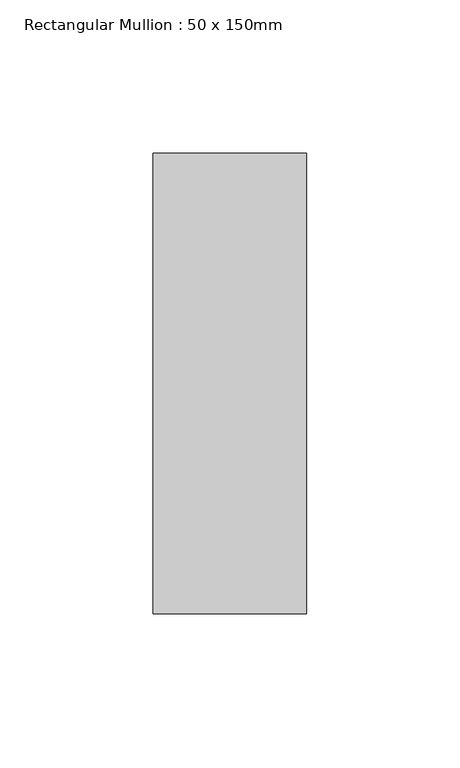
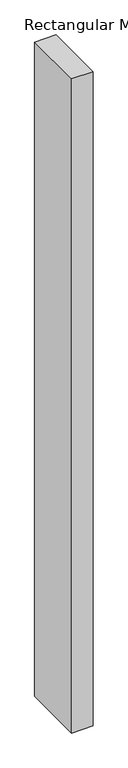
"""IFC4 building model written with IfcOpenShell, lengths in millimetres: member geometry, Rectangular Mullion : 50 x 150mm."""

import ifcopenshell
import ifcopenshell.guid

model = None  # the IFC model being written
_history = None  # IfcOwnerHistory: only IFC2X3 demands one
_inside = {}  # id of a spatial element -> (the spatial element, [elements in it])
_under = {}  # id of a project, library or spatial element -> (it, [spatial elements below it])
_declared = {}  # id of a project -> (the project, [libraries it declares])
_typed = {}  # id of a type object -> (the type object, [elements of that type])
_made_of = {}  # id of a material, layer set ... -> (it, [elements and type objects made of it])


def new_model(schema):
    """Start an empty IFC model of exactly this schema.

    Asked for "IFC4X3", IfcOpenShell would pick the latest addendum, in which some entities
    have other attributes; the version numbers below select the first issue.
    IFC2X3 requires an IfcOwnerHistory on every rooted entity: one is made here for all.
    """
    global model, _history
    if schema == "IFC4X3":
        model = ifcopenshell.file(schema_version=(4, 3, 0, 0))
    else:
        model = ifcopenshell.file(schema=schema)
    _inside.clear()
    _under.clear()
    _declared.clear()
    _typed.clear()
    _made_of.clear()
    _history = None
    if model.schema == "IFC2X3":
        org = make("IfcOrganization", Name="unknown")
        user = make(
            "IfcPersonAndOrganization",
            ThePerson=make("IfcPerson", FamilyName="unknown"),
            TheOrganization=org,
        )
        app = make(
            "IfcApplication",
            ApplicationDeveloper=org,
            Version="unknown",
            ApplicationFullName="unknown",
            ApplicationIdentifier="unknown",
        )
        _history = make(
            "IfcOwnerHistory",
            OwningUser=user,
            OwningApplication=app,
            ChangeAction="ADDED",
            CreationDate=0,
        )
    return model


def make(cls, **values):
    """One entity of the class cls with the attributes given. An attribute that is None is left unset."""
    return model.create_entity(
        cls, **{name: value for name, value in values.items() if value is not None}
    )


def rooted(cls, **values):
    """An entity with a GlobalId (a new one), such as an element, a storey or a relation."""
    return make(cls, GlobalId=ifcopenshell.guid.new(), OwnerHistory=_history, **values)


def si_unit(unit_type, name, prefix=None):
    """IfcSIUnit, for example si_unit("LENGTHUNIT", "METRE", prefix="MILLI")."""
    return make("IfcSIUnit", UnitType=unit_type, Prefix=prefix, Name=name)


def assignment(units):
    """IfcUnitAssignment: the units of a project."""
    return None if units is None else make("IfcUnitAssignment", Units=units)


def point(xyz):
    """IfcCartesianPoint."""
    return None if xyz is None else make("IfcCartesianPoint", Coordinates=xyz)


def direction(xyz):
    """IfcDirection."""
    return None if xyz is None else make("IfcDirection", DirectionRatios=xyz)


def frame(location, z_axis=None, x_axis=None):
    """IfcAxis2Placement3D, a coordinate frame: its origin and axes. An axis left out is left unset."""
    return make(
        "IfcAxis2Placement3D",
        Location=point(location),
        Axis=direction(z_axis),
        RefDirection=direction(x_axis),
    )


def origin():
    """The frame at (0, 0, 0) with its axes left unset."""
    return frame((0.0, 0.0, 0.0))


def place(relative_to, where):
    """IfcLocalPlacement: puts the frame where relative to a parent placement (None: the world)."""
    return make(
        "IfcLocalPlacement", PlacementRelTo=relative_to, RelativePlacement=where
    )


def context(
    kind, dimensions, precision=None, world=None, true_north=None, identifier=None
):
    """IfcGeometricRepresentationContext, for example the 3D "Model" context."""
    return make(
        "IfcGeometricRepresentationContext",
        ContextIdentifier=identifier,
        ContextType=kind,
        CoordinateSpaceDimension=dimensions,
        Precision=precision,
        WorldCoordinateSystem=world,
        TrueNorth=true_north,
    )


def project(units=None, contexts=None):
    """IfcProject with its units and contexts."""
    return rooted(
        "IfcProject",
        Name="project",
        RepresentationContexts=contexts,
        UnitsInContext=assignment(units),
    )


def spatial(cls, under=None, at=None, **own):
    """A site, building, storey or space (cls), placed at a placement, below another one or the project."""
    s = rooted(cls, ObjectPlacement=at, **own)
    if under is not None:
        _under.setdefault(under.id(), (under, []))[1].append(s)
    return s


def polyline(points):
    """IfcPolyline through the points."""
    return make("IfcPolyline", Points=[point(p) for p in points])


def outline(outer, holes=None, kind="AREA"):
    """IfcArbitraryClosedProfileDef: a profile drawn as a closed curve; with holes, ...WithVoids."""
    if holes is None:
        return make("IfcArbitraryClosedProfileDef", ProfileType=kind, OuterCurve=outer)
    return make(
        "IfcArbitraryProfileDefWithVoids",
        ProfileType=kind,
        OuterCurve=outer,
        InnerCurves=holes,
    )


def extrude(swept, where, along, depth):
    """IfcExtrudedAreaSolid: the profile swept, set in the frame where, extruded along a direction by depth."""
    return make(
        "IfcExtrudedAreaSolid",
        SweptArea=swept,
        Position=where,
        ExtrudedDirection=direction(along),
        Depth=depth,
    )


def shape(context_of_items, identifier, shape_type, items):
    """IfcShapeRepresentation: the items that make up one representation, for example the "Body"."""
    return make(
        "IfcShapeRepresentation",
        ContextOfItems=context_of_items,
        RepresentationIdentifier=identifier,
        RepresentationType=shape_type,
        Items=items,
    )


def source(mapping_origin, context_of_items, identifier, shape_type, items):
    """IfcRepresentationMap: a shape defined once, which mapped items show again and again."""
    return make(
        "IfcRepresentationMap",
        MappingOrigin=mapping_origin,
        MappedRepresentation=shape(context_of_items, identifier, shape_type, items),
    )


def transform(
    local_origin,
    x_axis=None,
    y_axis=None,
    z_axis=None,
    scale=None,
    scale2=None,
    scale3=None,
    uniform=True,
):
    """IfcCartesianTransformationOperator3D, or its non-uniform kind. x_axis, y_axis, z_axis: its Axis1, 2, 3."""
    if uniform:
        return make(
            "IfcCartesianTransformationOperator3D",
            Axis1=direction(x_axis),
            Axis2=direction(y_axis),
            LocalOrigin=point(local_origin),
            Scale=scale,
            Axis3=direction(z_axis),
        )
    return make(
        "IfcCartesianTransformationOperator3DnonUniform",
        Axis1=direction(x_axis),
        Axis2=direction(y_axis),
        LocalOrigin=point(local_origin),
        Scale=scale,
        Axis3=direction(z_axis),
        Scale2=scale2,
        Scale3=scale3,
    )


def mapped(mapping_source, mapping_target):
    """IfcMappedItem: shows the shape of a source again, moved by a transform."""
    return make(
        "IfcMappedItem", MappingSource=mapping_source, MappingTarget=mapping_target
    )


def made_of(thing, what):
    """Note that an element or type object is made of a material, layer set ...; save() writes the relation."""
    if what is not None:
        _made_of.setdefault(what.id(), (what, []))[1].append(thing)
    return thing


def element(
    cls,
    number,
    at=None,
    inside=None,
    cuts=None,
    type_object=None,
    material=None,
    context=None,
    identifier="Body",
    shape_type=None,
    held_by="IfcProductDefinitionShape",
    body=None,
    shapes=None,
    **own,
):
    """One element of the class cls, such as IfcWall. Its Tag is "e" and its number.

    at: its placement. inside: the storey or other place that contains it. cuts: it is an
    opening in that element (IfcRelVoidsElement). A single representation is given by context,
    identifier, shape_type and body (its items); several are given by shapes. held_by: the class
    of the entity that holds the representations. save() writes the other relations.
    """
    e = rooted(cls, Tag="e%d" % number, ObjectPlacement=at, **own)
    if body is not None:
        shapes = [shape(context, identifier, shape_type, body)]
    if shapes is not None:
        e.Representation = make(held_by, Representations=shapes)
    if inside is not None:
        _inside.setdefault(inside.id(), (inside, []))[1].append(e)
    if cuts is not None:
        rooted(
            "IfcRelVoidsElement", RelatingBuildingElement=cuts, RelatedOpeningElement=e
        )
    if type_object is not None:
        _typed.setdefault(type_object.id(), (type_object, []))[1].append(e)
    return made_of(e, material)


def aggregate(whole, parts):
    """IfcRelAggregates: a whole, such as a stair, and the parts it consists of."""
    return rooted("IfcRelAggregates", RelatingObject=whole, RelatedObjects=parts)


def save(model, path):
    """Write the relations noted so far, then the file.

    IfcRelAggregates (storeys below a building ...), IfcRelContainedInSpatialStructure (elements
    in a storey), IfcRelDefinesByType, IfcRelAssociatesMaterial and IfcRelDeclares: one each for
    every whole, place, type object, material and project.
    """
    for whole, parts in _under.values():
        aggregate(whole, parts)
    for where, things in _inside.values():
        rooted(
            "IfcRelContainedInSpatialStructure",
            RelatedElements=things,
            RelatingStructure=where,
        )
    for kind, things in _typed.values():
        rooted("IfcRelDefinesByType", RelatedObjects=things, RelatingType=kind)
    for what, things in _made_of.values():
        rooted("IfcRelAssociatesMaterial", RelatedObjects=things, RelatingMaterial=what)
    for by, libraries in _declared.values():
        rooted("IfcRelDeclares", RelatingContext=by, RelatedDefinitions=libraries)
    model.write(path)


def rectangular_mullion_50_x_150mm_f3b243f3(model_context):
    return source(origin(), model_context, "Body", "SweptSolid", [
        extrude(outline(polyline([(25.0, 75.0), (25.0, -75.0), (-25.0, -75.0), (-25.0, 75.0), (25.0, 75.0)])), frame((0.0, 0.0, -1615.0), z_axis=(0.0, 0.0, 1.0), x_axis=(1.0, 0.0, 0.0)), (0.0, 0.0, 1.0), 1615.0),
    ])


if __name__ == "__main__":
    model = new_model("IFC4")
    model_context = context("Model", 3, world=origin())
    ifc_project = project(units=[si_unit("LENGTHUNIT", "METRE", prefix="MILLI")], contexts=[model_context])
    site = spatial("IfcSite", under=ifc_project)
    building = spatial("IfcBuilding", under=site)
    placement = place(None, origin())
    rectangular_mullion_50_x_150mm_shape = rectangular_mullion_50_x_150mm_f3b243f3(model_context)
    element("IfcMember", 1, ObjectType="Rectangular Mullion : 50 x 150mm", at=placement, inside=building, context=model_context, shape_type="MappedRepresentation", body=[
        mapped(rectangular_mullion_50_x_150mm_shape, transform((0.0, 0.0, 0.0), x_axis=(1.0, 0.0, 0.0), y_axis=(0.0, 1.0, 0.0), z_axis=(0.0, 0.0, 1.0))),
    ])
    save(model, "model.ifc")

# Revit data of these elements
# Type "Rectangular Mullion : 50 x 150mm"
#   built-in parameter 1007304 = 0.492126 (stored number, unit not read)
#   built-in parameter 1007301 = 0.082021 (stored number, unit not read)
#   built-in parameter 1007300 = 0.082021 (stored number, unit not read)
# Element 1 (IfcMember, "Rectangular Mullion : 50 x 150mm")
#   Materials on its faces: "Metal - Aluminium"
# Materials
#   "Metal - Aluminium": class "Metal", colour RGB 247 247 247, transparency 0
